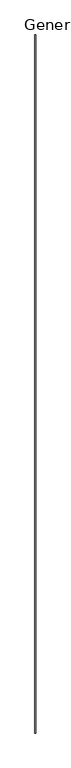
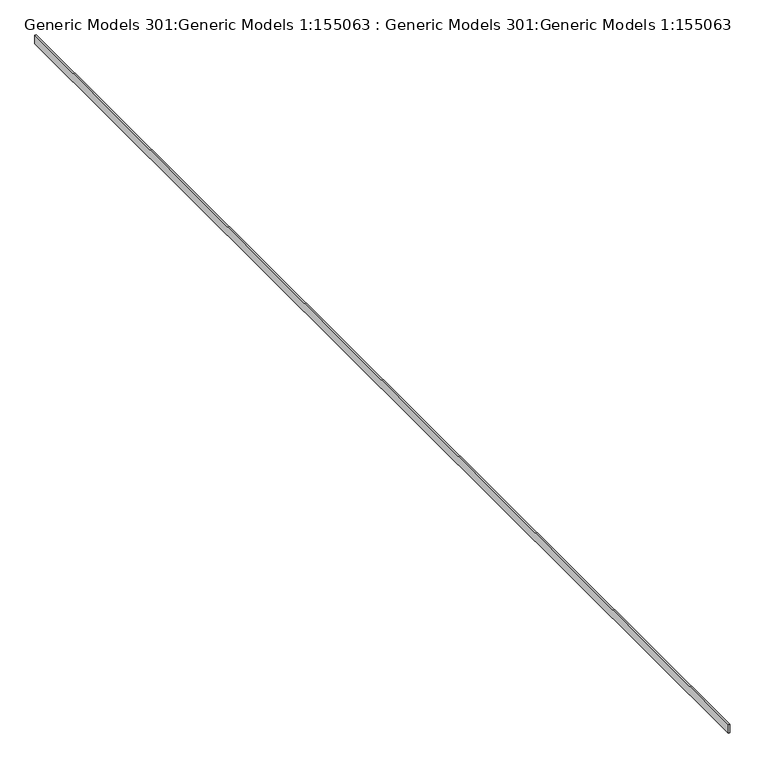
"""IFC4 building model written with IfcOpenShell, lengths in millimetres: proxy geometry, Generic Models 301:Generic Models 1:155063 : Generic Models 301:Generic Models 1:155063."""

from ifc_helpers import new_model, si_unit, frame, origin, place, context, project, spatial, polyline, outline, extrude, source, transform, mapped, element, save


def generic_models_301_generic_models_1_155063_generic_models_243e363f(model_context):
    return source(origin(), model_context, "Body", "SweptSolid", [
        extrude(outline(polyline([(165.1, 6652.5952178), (304.8, 6652.5952178), (304.8, 6634.7358428), (303.609375, 6633.5452178), (165.1, 6633.5452178), (165.1, 6652.5952178)])), frame((0.0, 8404.9928291, 0.0), z_axis=(0.0, 1.0, 0.0), x_axis=(0.0, 0.0, 1.0)), (0.0, 0.0, 1.0), 19050.0),
    ])


if __name__ == "__main__":
    model = new_model("IFC4")
    model_context = context("Model", 3, world=origin())
    ifc_project = project(units=[si_unit("LENGTHUNIT", "METRE", prefix="MILLI")], contexts=[model_context])
    site = spatial("IfcSite", under=ifc_project)
    building = spatial("IfcBuilding", under=site)
    placement = place(None, origin())
    generic_models_301_generic_models_1_155063_generic_models_shape = generic_models_301_generic_models_1_155063_generic_models_243e363f(model_context)
    element("IfcBuildingElementProxy", 1, Name="Generic Models 301:Generic Models 1:155063 : Generic Models 301:Generic Models 1:155063", ObjectType="Generic Models 301:Generic Models 1:155063 : Generic Models 301:Generic Models 1:155063", at=placement, inside=building, context=model_context, shape_type="MappedRepresentation", body=[
        mapped(generic_models_301_generic_models_1_155063_generic_models_shape, transform((0.0, 0.0, 0.0), x_axis=(1.0, 0.0, 0.0), y_axis=(0.0, 1.0, 0.0), z_axis=(0.0, 0.0, 1.0))),
    ])
    save(model, "model.ifc")

# Revit data of these elements
# Type "Generic Models 301:Generic Models 1:155063 : Generic Models 301:Generic Models 1:155063"
#   NameOverride = "Generic Models 301:Generic Models 1:155063"
#   ObjectTypeOverride = "Generic Models 301:Generic Models 1"
#   Reference = "Generic Models 1"
#   Category = "Generic Models"
#   Tag = "155063"
# Element 1 (IfcBuildingElementProxy, "Generic Models 301:Generic Models 1:155063 : Generic Models 301:Generic Models 1:155063")
#   Materials on its faces: "_BASE TRIM AS SCHEDULED 29642"
# Materials
#   "_BASE TRIM AS SCHEDULED 29642": class "Unassigned", colour RGB 177 130 114, transparency 0
